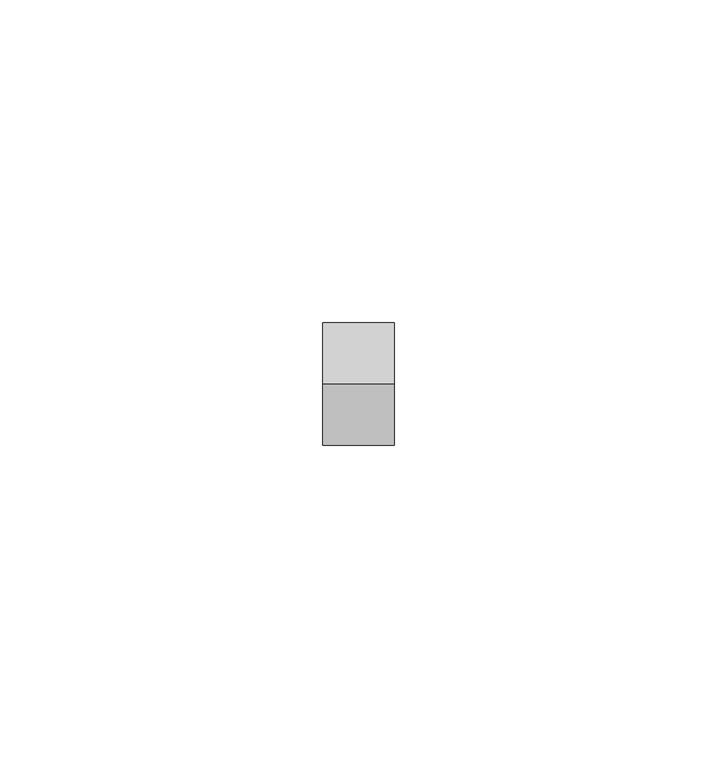
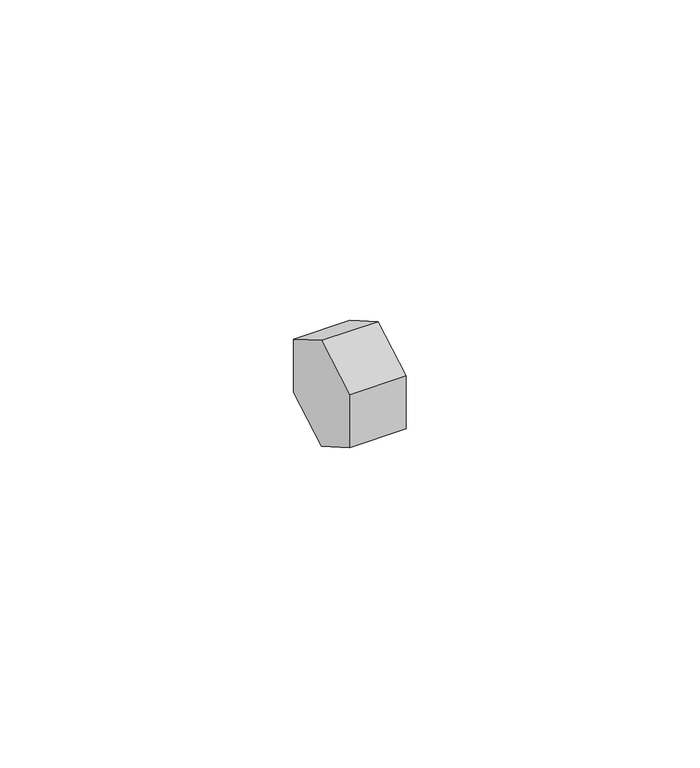
"""IFC4 building model written with IfcOpenShell, lengths in millimetres: proxy geometry, Generic Models 7:Generic Models 1:8:Generic Models 1:8 : Generic Models 7:Generic Models 1:337419:13 : Generic Models 7:Generic Models 1:8:Generic Models 1:8 : Generic Models 7:Generic Models 1:337419:315935."""

from ifc_helpers import new_model, si_unit, frame, origin, place, context, project, spatial, polyline, outline, extrude, source, transform, mapped, element, save


def generic_models_5d3ef85f(model_context):
    return source(origin(), model_context, "Body", "SweptSolid", [
        extrude(outline(polyline([(-564919.104849, 8833.512141), (-564928.629849, 8839.0114023), (-564928.629849, 8850.009925), (-564919.104849, 8855.5091863), (-564909.579849, 8850.009925), (-564909.579849, 8839.0114023), (-564919.104849, 8833.512141)])), frame((593804.563286, 0.0, 0.0), z_axis=(1.0, 0.0, 0.0), x_axis=(0.0, 1.0, 0.0)), (0.0, 0.0, 1.0), 11.1125),
    ])


if __name__ == "__main__":
    model = new_model("IFC4")
    model_context = context("Model", 3, world=origin())
    ifc_project = project(units=[si_unit("LENGTHUNIT", "METRE", prefix="MILLI")], contexts=[model_context])
    site = spatial("IfcSite", under=ifc_project)
    building = spatial("IfcBuilding", under=site)
    placement = place(None, origin())
    generic_models_shape = generic_models_5d3ef85f(model_context)
    element("IfcBuildingElementProxy", 1, Name="Generic Models 7:Generic Models 1:8:Generic Models 1:8 : Generic Models 7:Generic Models 1:337419:13 : Generic Models 7:Generic Models 1:8:Generic Models 1:8 : Generic Models 7:Generic Models 1:337419:315935", ObjectType="Generic Models 7:Generic Models 1:8:Generic Models 1:8 : Generic Models 7:Generic Models 1:337419:13 : Generic Models 7:Generic Models 1:8:Generic Models 1:8 : Generic Models 7:Generic Models 1:337419:315935", at=placement, inside=building, context=model_context, shape_type="MappedRepresentation", body=[
        mapped(generic_models_shape, transform((0.0, 0.0, 0.0), x_axis=(1.0, 0.0, 0.0), y_axis=(0.0, 1.0, 0.0), z_axis=(0.0, 0.0, 1.0))),
    ])
    save(model, "model.ifc")

# Revit data of these elements
# Type "Generic Models 7:Generic Models 1:8:Generic Models 1:8 : Generic Models 7:Generic Models 1:337419:13 : Generic Models 7:Generic Models 1:8:Generic Models 1:8 : Generic Models 7:Generic Models 1:337419:315935"
#   NameOverride = "Generic Models 7:Generic Models 1:8:Generic Models 1:8 : Generic Models 7:Generic Models 1:337419:315935"
#   ObjectTypeOverride = "Generic Models 1:8 : Generic Models 7:Generic Models 1:337419"
#   Reference = "Generic Models 1"
#   Tag = "315935"
# Element 1 (IfcBuildingElementProxy, "Generic Models 7:Generic Models 1:8:Generic Models 1:8 : Generic Models 7:Generic Models 1:337419:13 : Generic Models 7:Generic Models 1:8:Generic Models 1:8 : Generic Models 7:Generic Models 1:337419:315935")
#   Materials on its faces: "1/2\" THRU BOLTS"
# Materials
#   "1/2\" THRU BOLTS": class "Generic", colour RGB 120 120 120, transparency 0, Cost = 0
